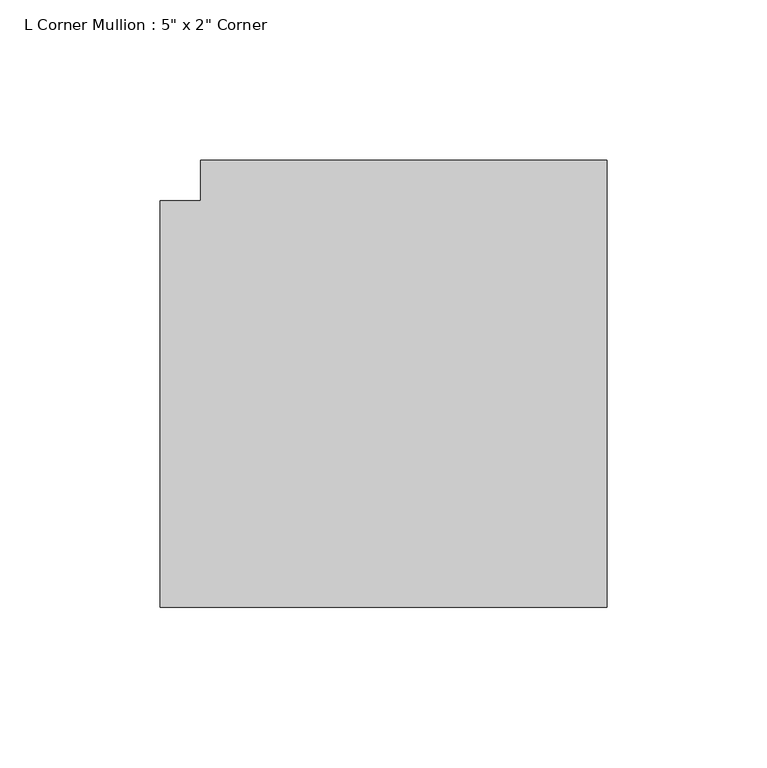
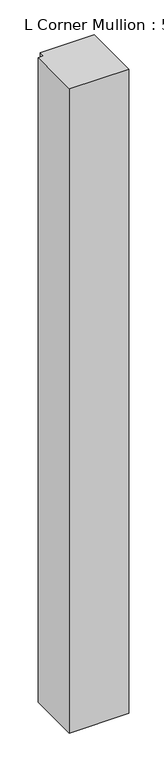
"""IFC4 building model written with IfcOpenShell, lengths in millimetres: member geometry."""

from ifc_helpers import new_model, si_unit, frame, origin, place, context, project, spatial, polyline, outline, extrude, source, transform, mapped, element, save


def member_5b126e42(model_context):
    return source(origin(), model_context, "Body", "SweptSolid", [
        extrude(outline(polyline([(63.5, 76.2), (63.5, -63.5), (-76.2, -63.5), (-76.2, 63.5), (-63.5, 63.5), (-63.5, 76.2), (63.5, 76.2)])), frame((0.0, 0.0, -1600.2), z_axis=(0.0, 0.0, 1.0), x_axis=(1.0, 0.0, 0.0)), (0.0, 0.0, 1.0), 1600.2),
    ])


if __name__ == "__main__":
    model = new_model("IFC4")
    model_context = context("Model", 3, world=origin())
    ifc_project = project(units=[si_unit("LENGTHUNIT", "METRE", prefix="MILLI")], contexts=[model_context])
    site = spatial("IfcSite", under=ifc_project)
    building = spatial("IfcBuilding", under=site)
    placement = place(None, origin())
    member_shape = member_5b126e42(model_context)
    element("IfcMember", 1, ObjectType="L Corner Mullion : 5\" x 2\" Corner", at=placement, inside=building, context=model_context, shape_type="MappedRepresentation", body=[
        mapped(member_shape, transform((0.0, 0.0, 0.0), x_axis=(1.0, 0.0, 0.0), y_axis=(0.0, 1.0, 0.0), z_axis=(0.0, 0.0, 1.0))),
    ])
    save(model, "model.ifc")

# Revit data of these elements
# Type "L Corner Mullion : 5\" x 2\" Corner"
#   built-in parameter 1007355 = 0.25 (stored number, unit not read)
#   built-in parameter 1007354 = 0.25 (stored number, unit not read)
#   built-in parameter 1007304 = 0.416667 (stored number, unit not read)
# Element 1 (IfcMember, "L Corner Mullion : 5\" x 2\" Corner")
#   Materials on its faces: "Metal - Aluminum"
# Materials
#   "Metal - Aluminum": class "Metal", colour RGB 109 108 108, transparency 0
